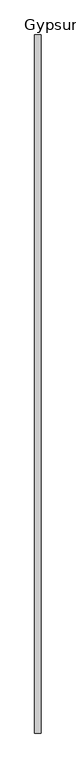
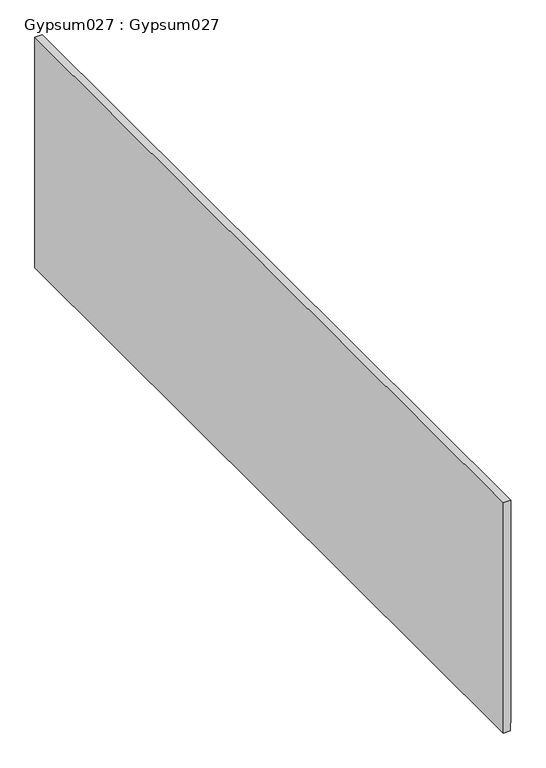
"""IFC4 building model written with IfcOpenShell, lengths in millimetres: proxy geometry, Gypsum027 : Gypsum027."""

from ifc_helpers import new_model, si_unit, frame, origin, place, context, project, spatial, polyline, outline, extrude, source, transform, mapped, element, save


def gypsum027_gypsum027_bfbcf28b(model_context):
    return source(origin(), model_context, "Body", "SweptSolid", [
        extrude(outline(polyline([(35656.0216362, -8269.6582011), (35055.7176364, -8269.6582011), (35055.7176364, -8253.1630283), (35076.8706722, -8253.1630283), (35076.8706722, -8251.8779965), (35656.0216362, -8251.8779965), (35656.0216362, -8269.6582011)])), frame((0.0, 4540.4513986, 0.0), z_axis=(0.0, 1.0, 0.0), x_axis=(0.0, 0.0, 1.0)), (0.0, 0.0, 1.0), 2000.0),
    ])


if __name__ == "__main__":
    model = new_model("IFC4")
    model_context = context("Model", 3, world=origin())
    ifc_project = project(units=[si_unit("LENGTHUNIT", "METRE", prefix="MILLI")], contexts=[model_context])
    site = spatial("IfcSite", under=ifc_project)
    building = spatial("IfcBuilding", under=site)
    placement = place(None, origin())
    gypsum027_gypsum027_shape = gypsum027_gypsum027_bfbcf28b(model_context)
    element("IfcBuildingElementProxy", 1, Name="Gypsum027 : Gypsum027", ObjectType="Gypsum027 : Gypsum027", at=placement, inside=building, context=model_context, shape_type="MappedRepresentation", body=[
        mapped(gypsum027_gypsum027_shape, transform((0.0, 0.0, 0.0), x_axis=(1.0, 0.0, 0.0), y_axis=(0.0, 1.0, 0.0), z_axis=(0.0, 0.0, 1.0))),
    ])
    save(model, "model.ifc")

# Revit data of these elements
# Type "Gypsum027 : Gypsum027"
#   NameOverride = "Gypsum027"
# Element 1 (IfcBuildingElementProxy, "Gypsum027 : Gypsum027")
#   Materials on its faces: "5/8\" GYPSUM BOARD"
# Materials
#   "5/8\" GYPSUM BOARD": class "Unassigned", colour RGB 214 214 214, transparency 0, Cost = 0
